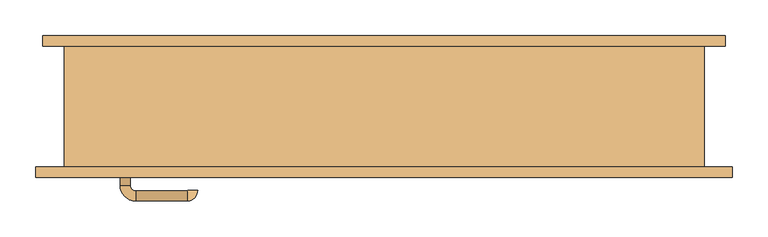
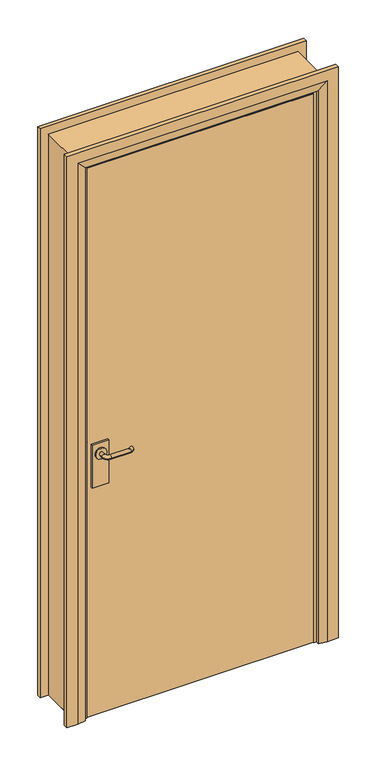
"""IFC4 building model written with IfcOpenShell, lengths in millimetres: door geometry, Porta Simples de Abrir : 80x210cm - Marco de Madeira."""

from ifc_helpers import new_model, si_unit, point, frame, frame_2d, origin, place, context, project, spatial, polyline, circle_curve, ellipse_curve, trimmed, segment, composite_curve, outline, extrude, faceted_brep, source, transform, mapped, element, save
from ifc_brep_helpers import plane_surface, cylinder_surface, revolved_surface, advanced_brep


def door_78011655(model_context):
    return source(origin(), model_context, "Body", "SolidModel", [
        extrude(outline(composite_curve([segment(trimmed(circle_curve(frame_2d((1050.0, -364.0)), 20.0), [point((1050.0, -384.0))], [point((1050.0, -344.0))], False, "CARTESIAN"), True, "CONTINUOUS"), segment(trimmed(circle_curve(frame_2d((1050.0, -364.0)), 20.0), [point((1050.0, -344.0))], [point((1050.0, -384.0))], False, "CARTESIAN"), True, "CONTINUOUS")], self_intersect=False)), frame((0.0, -44.0, 0.0), z_axis=(0.0, 1.0, 0.0), x_axis=(0.0, 0.0, 1.0)), (0.0, 0.0, 1.0), 4.5929895),
        advanced_brep(
        [(-357.0, -39.4070105, 1050.0), (-371.0, -39.4070105, 1050.0), (-357.0, -24.0, 1050.0), (-371.0, -24.0, 1050.0), (-349.0, -2.0, 1050.0), (-349.0, -16.0, 1050.0), (-277.0, -16.0, 1050.0), (-277.0, -2.0, 1050.0), (-276.0, -17.0, 1050.0), (-262.0, -17.0, 1050.0)],
        [
            (0, 1, circle_curve(frame((-364.0, -39.4070105, 1050.0), z_axis=(0.0, -1.0, 0.0), x_axis=(-1.0, 0.0, 0.0)), 7.0)),
            (1, 0, circle_curve(frame((-364.0, -39.4070105, 1050.0), z_axis=(0.0, -1.0, 0.0), x_axis=(-1.0, 0.0, 0.0)), 7.0)),
            (0, 2),
            (2, 3, circle_curve(frame((-364.0, -24.0, 1050.0), z_axis=(0.0, -1.0, 0.0), x_axis=(-1.0, 0.0, 0.0)), 7.0)),
            (3, 1),
            (3, 2, circle_curve(frame((-364.0, -24.0, 1050.0), z_axis=(0.0, -1.0, 0.0), x_axis=(-1.0, 0.0, 0.0)), 7.0)),
            (4, 3, circle_curve(frame((-349.0, -24.0, 1050.0), z_axis=(0.0, 0.0, 1.0), x_axis=(-1.0, 0.0, 0.0)), 22.0)),
            (2, 5, circle_curve(frame((-349.0, -24.0, 1050.0), z_axis=(0.0, 0.0, -1.0), x_axis=(-1.0, 0.0, 0.0)), 8.0)),
            (5, 4, circle_curve(frame((-349.0, -9.0, 1050.0), z_axis=(-1.0, 0.0, 0.0), x_axis=(0.0, 1.0, 0.0)), 7.0)),
            (4, 5, circle_curve(frame((-349.0, -9.0, 1050.0), z_axis=(-1.0, 0.0, 0.0), x_axis=(0.0, 1.0, 0.0)), 7.0)),
            (5, 6),
            (6, 7, circle_curve(frame((-277.0, -9.0, 1050.0), z_axis=(-1.0, 0.0, 0.0), x_axis=(0.0, 1.0, 0.0)), 7.0)),
            (7, 4),
            (7, 6, circle_curve(frame((-277.0, -9.0, 1050.0), z_axis=(-1.0, 0.0, 0.0), x_axis=(0.0, 1.0, 0.0)), 7.0)),
            (8, 9, circle_curve(frame((-269.0, -17.0, 1050.0), z_axis=(0.0, -1.0, 0.0), x_axis=(1.0, 0.0, 0.0)), 7.0)),
            (9, 8, circle_curve(frame((-269.0, -17.0, 1050.0), z_axis=(0.0, -1.0, 0.0), x_axis=(1.0, 0.0, 0.0)), 7.0)),
            (9, 7, circle_curve(frame((-277.0, -17.0, 1050.0), z_axis=(0.0, 0.0, 1.0), x_axis=(0.0, 1.0, 0.0)), 15.0)),
            (6, 8, circle_curve(frame((-277.0, -17.0, 1050.0), z_axis=(0.0, 0.0, -1.0), x_axis=(0.0, 1.0, 0.0)), 1.0)),
        ],
        [
            plane_surface(frame((-364.0, -39.4070105, 1050.0), z_axis=(0.0, -1.0, 0.0), x_axis=(0.0, 0.0, 1.0))),
            cylinder_surface(frame((-364.0, -39.4070105, 1050.0), z_axis=(0.0, -1.0, 0.0), x_axis=(-1.0, 0.0, 0.0)), 7.0),
            revolved_surface(trimmed(ellipse_curve(frame((-364.0, -24.0, 1050.0), z_axis=(0.0, -1.0, 0.0), x_axis=(-1.0, 0.0, 0.0)), 7.0, 7.0), [point((-357.0, -24.0, 1050.0))], [point((-371.0, -24.0, 1050.0))], True, "CARTESIAN"), (-349.0, -24.0, 1050.0), (0.0, 0.0, -1.0)),
            revolved_surface(trimmed(ellipse_curve(frame((-364.0, -24.0, 1050.0), z_axis=(0.0, -1.0, 0.0), x_axis=(-1.0, 0.0, 0.0)), 7.0, 7.0), [point((-371.0, -24.0, 1050.0))], [point((-357.0, -24.0, 1050.0))], True, "CARTESIAN"), (-349.0, -24.0, 1050.0), (0.0, 0.0, -1.0)),
            cylinder_surface(frame((-349.0, -9.0, 1050.0), z_axis=(-1.0, 0.0, 0.0), x_axis=(0.0, 1.0, 0.0)), 7.0),
            plane_surface(frame((-269.0, -17.0, 1050.0), z_axis=(0.0, -1.0, 0.0), x_axis=(0.0, 0.0, 1.0))),
            revolved_surface(trimmed(ellipse_curve(frame((-277.0, -9.0, 1050.0), z_axis=(-1.0, 0.0, 0.0), x_axis=(0.0, 1.0, 0.0)), 7.0, 7.0), [point((-277.0, -16.0, 1050.0))], [point((-277.0, -2.0, 1050.0))], True, "CARTESIAN"), (-277.0, -17.0, 1050.0), (0.0, 0.0, -1.0)),
            revolved_surface(trimmed(ellipse_curve(frame((-277.0, -9.0, 1050.0), z_axis=(-1.0, 0.0, 0.0), x_axis=(0.0, 1.0, 0.0)), 7.0, 7.0), [point((-277.0, -2.0, 1050.0))], [point((-277.0, -16.0, 1050.0))], True, "CARTESIAN"), (-277.0, -17.0, 1050.0), (0.0, 0.0, -1.0)),
        ],
        [
            (0, [[1, 2]]),
            (1, [[-1, 3, 4, 5]]),
            (1, [[-2, -5, 6, -3]]),
            (2, [[7, -4, 8, 9]]),
            (3, [[-8, -6, -7, 10]]),
            (4, [[-9, 11, 12, 13]]),
            (4, [[-10, -13, 14, -11]]),
            (5, [[15, 16]]),
            (6, [[17, -12, 18, -16]]),
            (7, [[-18, -14, -17, -15]]),
        ],
    ),
        extrude(outline(polyline([(-334.0, -50.0), (-394.0, -50.0), (-394.0, -44.0), (-334.0, -44.0), (-334.0, -50.0)])), frame((0.0, 0.0, 925.0), z_axis=(0.0, 0.0, 1.0), x_axis=(1.0, 0.0, 0.0)), (0.0, 0.0, 1.0), 165.0),
        extrude(outline(composite_curve([segment(trimmed(circle_curve(frame_2d((1050.0, -364.0)), 20.0), [point((1050.0, -384.0))], [point((1050.0, -344.0))], False, "CARTESIAN"), True, "CONTINUOUS"), segment(trimmed(circle_curve(frame_2d((1050.0, -364.0)), 20.0), [point((1050.0, -344.0))], [point((1050.0, -384.0))], False, "CARTESIAN"), True, "CONTINUOUS")], self_intersect=False)), frame((0.0, -95.5929895, 0.0), z_axis=(0.0, 1.0, 0.0), x_axis=(0.0, 0.0, 1.0)), (0.0, 0.0, 1.0), 4.5929895),
        advanced_brep(
        [(-357.0, -95.5929895, 1050.0), (-371.0, -95.5929895, 1050.0), (-371.0, -111.0, 1050.0), (-357.0, -111.0, 1050.0), (-349.0, -133.0, 1050.0), (-349.0, -119.0, 1050.0), (-277.0, -133.0, 1050.0), (-277.0, -119.0, 1050.0), (-276.0, -118.0, 1050.0), (-262.0, -118.0, 1050.0)],
        [
            (0, 1, circle_curve(frame((-364.0, -95.5929895, 1050.0), z_axis=(0.0, 1.0, 0.0), x_axis=(-1.0, 0.0, 0.0)), 7.0)),
            (1, 0, circle_curve(frame((-364.0, -95.5929895, 1050.0), z_axis=(0.0, 1.0, 0.0), x_axis=(-1.0, 0.0, 0.0)), 7.0)),
            (1, 2),
            (2, 3, circle_curve(frame((-364.0, -111.0, 1050.0), z_axis=(0.0, 1.0, 0.0), x_axis=(-1.0, 0.0, 0.0)), 7.0)),
            (3, 0),
            (3, 2, circle_curve(frame((-364.0, -111.0, 1050.0), z_axis=(0.0, 1.0, 0.0), x_axis=(-1.0, 0.0, 0.0)), 7.0)),
            (4, 5, circle_curve(frame((-349.0, -126.0, 1050.0), z_axis=(-1.0, 0.0, 0.0), x_axis=(0.0, -1.0, 0.0)), 7.0)),
            (5, 3, circle_curve(frame((-349.0, -111.0, 1050.0), z_axis=(0.0, 0.0, -1.0), x_axis=(-1.0, 0.0, 0.0)), 8.0)),
            (2, 4, circle_curve(frame((-349.0, -111.0, 1050.0), z_axis=(0.0, 0.0, 1.0), x_axis=(-1.0, 0.0, 0.0)), 22.0)),
            (5, 4, circle_curve(frame((-349.0, -126.0, 1050.0), z_axis=(-1.0, 0.0, 0.0), x_axis=(0.0, -1.0, 0.0)), 7.0)),
            (4, 6),
            (6, 7, circle_curve(frame((-277.0, -126.0, 1050.0), z_axis=(-1.0, 0.0, 0.0), x_axis=(0.0, -1.0, 0.0)), 7.0)),
            (7, 5),
            (7, 6, circle_curve(frame((-277.0, -126.0, 1050.0), z_axis=(-1.0, 0.0, 0.0), x_axis=(0.0, -1.0, 0.0)), 7.0)),
            (8, 9, circle_curve(frame((-269.0, -118.0, 1050.0), z_axis=(0.0, 1.0, 0.0), x_axis=(1.0, 0.0, 0.0)), 7.0)),
            (9, 8, circle_curve(frame((-269.0, -118.0, 1050.0), z_axis=(0.0, 1.0, 0.0), x_axis=(1.0, 0.0, 0.0)), 7.0)),
            (8, 7, circle_curve(frame((-277.0, -118.0, 1050.0), z_axis=(0.0, 0.0, -1.0), x_axis=(0.0, -1.0, 0.0)), 1.0)),
            (6, 9, circle_curve(frame((-277.0, -118.0, 1050.0), z_axis=(0.0, 0.0, 1.0), x_axis=(0.0, -1.0, 0.0)), 15.0)),
        ],
        [
            plane_surface(frame((-364.0, -95.5929895, 1050.0), z_axis=(0.0, 1.0, 0.0), x_axis=(0.0, 0.0, 1.0))),
            cylinder_surface(frame((-364.0, -95.5929895, 1050.0), z_axis=(0.0, 1.0, 0.0), x_axis=(-1.0, 0.0, 0.0)), 7.0),
            revolved_surface(trimmed(ellipse_curve(frame((-364.0, -111.0, 1050.0), z_axis=(0.0, -1.0, 0.0), x_axis=(-1.0, 0.0, 0.0)), 7.0, 7.0), [point((-357.0, -111.0, 1050.0))], [point((-371.0, -111.0, 1050.0))], True, "CARTESIAN"), (-349.0, -111.0, 1050.0), (0.0, 0.0, -1.0)),
            revolved_surface(trimmed(ellipse_curve(frame((-364.0, -111.0, 1050.0), z_axis=(0.0, -1.0, 0.0), x_axis=(-1.0, 0.0, 0.0)), 7.0, 7.0), [point((-371.0, -111.0, 1050.0))], [point((-357.0, -111.0, 1050.0))], True, "CARTESIAN"), (-349.0, -111.0, 1050.0), (0.0, 0.0, -1.0)),
            cylinder_surface(frame((-349.0, -126.0, 1050.0), z_axis=(-1.0, 0.0, 0.0), x_axis=(0.0, -1.0, 0.0)), 7.0),
            plane_surface(frame((-269.0, -118.0, 1050.0), z_axis=(0.0, 1.0, 0.0), x_axis=(0.0, 0.0, 1.0))),
            revolved_surface(trimmed(ellipse_curve(frame((-277.0, -126.0, 1050.0), z_axis=(1.0, 0.0, 0.0), x_axis=(0.0, -1.0, 0.0)), 7.0, 7.0), [point((-277.0, -119.0, 1050.0))], [point((-277.0, -133.0, 1050.0))], True, "CARTESIAN"), (-277.0, -118.0, 1050.0), (0.0, 0.0, -1.0)),
            revolved_surface(trimmed(ellipse_curve(frame((-277.0, -126.0, 1050.0), z_axis=(1.0, 0.0, 0.0), x_axis=(0.0, -1.0, 0.0)), 7.0, 7.0), [point((-277.0, -133.0, 1050.0))], [point((-277.0, -119.0, 1050.0))], True, "CARTESIAN"), (-277.0, -118.0, 1050.0), (0.0, 0.0, -1.0)),
        ],
        [
            (0, [[1, 2]]),
            (1, [[3, 4, 5, -2]]),
            (1, [[-5, 6, -3, -1]]),
            (2, [[7, 8, -4, 9]]),
            (3, [[10, -9, -6, -8]]),
            (4, [[11, 12, 13, -7]]),
            (4, [[-13, 14, -11, -10]]),
            (5, [[15, 16]]),
            (6, [[-15, 17, -12, 18]]),
            (7, [[-16, -18, -14, -17]]),
        ],
    ),
        extrude(outline(polyline([(-334.0, -85.0), (-334.0, -91.0), (-394.0, -91.0), (-394.0, -85.0), (-334.0, -85.0)])), frame((0.0, 0.0, 925.0), z_axis=(0.0, 0.0, 1.0), x_axis=(1.0, 0.0, 0.0)), (0.0, 0.0, 1.0), 165.0),
        extrude(outline(polyline([(408.0, -50.0), (408.0, -85.0), (-408.0, -85.0), (-408.0, -50.0), (408.0, -50.0)])), frame((0.0, 0.0, 53.0), z_axis=(0.0, 0.0, 1.0), x_axis=(1.0, 0.0, 0.0)), (0.0, 0.0, 1.0), 2094.0),
        faceted_brep([(480.0, 85.0, 50.0), (410.0, 85.0, 50.0), (410.0, 95.0, 50.0), (440.0, 100.0, 50.0), (480.0, 100.0, 50.0), (480.0, 100.0, 2220.0), (480.0, 85.0, 2220.0), (440.0, 100.0, 2180.0), (-440.0, 100.0, 2180.0), (-440.0, 100.0, 50.0), (-480.0, 100.0, 50.0), (-480.0, 100.0, 2220.0), (410.0, 95.0, 2150.0), (410.0, 85.0, 2150.0), (-480.0, 85.0, 2220.0), (-480.0, 85.0, 50.0), (-410.0, 85.0, 50.0), (-410.0, 85.0, 2150.0), (-410.0, 95.0, 50.0), (-410.0, 95.0, 2150.0)], [[[0, 1, 2, 3, 4]], [[4, 5, 6, 0]], [[3, 7, 8, 9, 10, 11, 5, 4]], [[2, 12, 7, 3]], [[1, 13, 12, 2]], [[0, 6, 14, 15, 16, 17, 13, 1]], [[17, 16, 18, 19]], [[15, 10, 9, 18, 16]], [[11, 10, 15, 14]], [[19, 18, 9, 8]], [[13, 17, 19, 12]], [[5, 11, 14, 6]], [[12, 19, 8, 7]]]),
        faceted_brep([(490.0, -85.0, 50.0), (490.0, -100.0, 50.0), (450.0, -100.0, 50.0), (420.0, -95.0, 50.0), (420.0, -85.0, 50.0), (420.0, -85.0, 2160.0), (-420.0, -85.0, 2160.0), (-420.0, -85.0, 50.0), (-490.0, -85.0, 50.0), (-490.0, -85.0, 2230.0), (490.0, -85.0, 2230.0), (420.0, -95.0, 2160.0), (450.0, -100.0, 2190.0), (490.0, -100.0, 2230.0), (-490.0, -100.0, 2230.0), (-490.0, -100.0, 50.0), (-450.0, -100.0, 50.0), (-450.0, -100.0, 2190.0), (-420.0, -95.0, 50.0), (-420.0, -95.0, 2160.0)], [[[0, 1, 2, 3, 4]], [[4, 5, 6, 7, 8, 9, 10, 0]], [[3, 11, 5, 4]], [[2, 12, 11, 3]], [[1, 13, 14, 15, 16, 17, 12, 2]], [[0, 10, 13, 1]], [[9, 8, 15, 14]], [[8, 7, 18, 16, 15]], [[19, 18, 7, 6]], [[17, 16, 18, 19]], [[11, 19, 6, 5]], [[10, 9, 14, 13]], [[12, 17, 19, 11]]]),
        faceted_brep([(-410.0, -85.0, 50.0), (-450.0, -85.0, 50.0), (-450.0, 85.0, 50.0), (-400.0, 85.0, 50.0), (-400.0, -48.0, 50.0), (-410.0, -48.0, 50.0), (-410.0, -48.0, 2150.0), (-410.0, -85.0, 2150.0), (-400.0, -48.0, 2140.0), (-400.0, 85.0, 2140.0), (-450.0, 85.0, 2190.0), (-450.0, -85.0, 2190.0), (410.0, -85.0, 50.0), (410.0, -48.0, 50.0), (400.0, -48.0, 50.0), (400.0, 85.0, 50.0), (450.0, 85.0, 50.0), (450.0, -85.0, 50.0), (410.0, -85.0, 2150.0), (450.0, -85.0, 2190.0), (450.0, 85.0, 2190.0), (400.0, 85.0, 2140.0), (400.0, -48.0, 2140.0), (410.0, -48.0, 2150.0)], [[[0, 1, 2, 3, 4, 5]], [[5, 6, 7, 0]], [[4, 8, 6, 5]], [[3, 9, 8, 4]], [[2, 10, 9, 3]], [[1, 11, 10, 2]], [[0, 7, 11, 1]], [[12, 13, 14, 15, 16, 17]], [[18, 12, 17, 19]], [[19, 17, 16, 20]], [[20, 16, 15, 21]], [[21, 15, 14, 22]], [[22, 14, 13, 23]], [[23, 13, 12, 18]], [[6, 23, 18, 7]], [[8, 22, 23, 6]], [[9, 21, 22, 8]], [[10, 20, 21, 9]], [[11, 19, 20, 10]], [[7, 18, 19, 11]]]),
        extrude(outline(polyline([(450.0, -50.0), (-450.0, -50.0), (-450.0, 85.0), (450.0, 85.0), (450.0, -50.0)])), frame((0.0, 0.0, 50.0), z_axis=(0.0, 0.0, 1.0), x_axis=(1.0, 0.0, 0.0)), (0.0, 0.0, 1.0), 3.0),
    ])


if __name__ == "__main__":
    model = new_model("IFC4")
    model_context = context("Model", 3, world=origin())
    ifc_project = project(units=[si_unit("LENGTHUNIT", "METRE", prefix="MILLI")], contexts=[model_context])
    site = spatial("IfcSite", under=ifc_project)
    building = spatial("IfcBuilding", under=site)
    placement = place(None, origin())
    door_shape = door_78011655(model_context)
    element("IfcDoor", 1, ObjectType="Porta Simples de Abrir : 80x210cm - Marco de Madeira", at=placement, inside=building, context=model_context, shape_type="MappedRepresentation", body=[
        mapped(door_shape, transform((0.0, 0.0, 0.0), x_axis=(1.0, 0.0, 0.0), y_axis=(0.0, 1.0, 0.0), z_axis=(0.0, 0.0, 1.0))),
    ])
    save(model, "model.ifc")

# Revit data of these elements
# Type "Porta Simples de Abrir : 80x210cm - Marco de Madeira"
#   Type Mark = "P57"
#   SINAPI = ""
#   Analytic Construction = "<Nenhum>"
#   Construction Type = "300"
#   Maçaneta [instance default] = ""
#   Fechadura [instance default] = ""
#   Vão Luz (somente para informação) = 0.780 m
#   Tolerância Folha Vertical = 0.003 m
#   Módulo Básico M = 0.100 m
#   Largura de Coordenação Modular Largura CM = 0.900 m
#   Rough Width = 0.900 m
#   Deslocamento da Horizontal da Folha = 0.000 m
#   Altura de Coordenação Modular Largura CM = 2.200 m
#   Rough Height = 2.200 m
#   Altura Nominal = 2.090 m
#   Ajuste de Coordenação Topo AC Topo = 0.010 m
#   Ajuste de Coordenação Base AC Base = 0.050 m
#   Ajuste de Coordenação AC = 0.010 m
#   Tolerância Folha Horizontal = 0.002 m
#   Largura Folha (somente para informação) = 0.796 m
#   Espessura Folha = 0.035 m
#   Maçaneta - Distância da Folha = 0.044 m
#   Maçaneta - Altura = 1.000 m
#   Largura Nominal (Largura Mn) = 0.820 m
#   Distância do Nível = 0.003 m
#   Aduela Interna Espessura = 0.040 m
#   Aduela Externa Espessura = 0.050 m
#   Altura Folha (somente para informação) = 2.075 m
#   Height = 2.140 m
#   Width = 0.880 m
#   Número de Módulos Básicos nM Largura = 9
#   Número de Módulos Básicos nM Altura = 22
#   Marco Metálico = no
#   Aduela de Madeira = no
#   Aduela Metálica de Canto = no
#   Guarnição Reta = no
#   Guarnição Chanfrada = yes
#   Batente - Material [instance default] = none
#   Painel - Material [instance default] = none
#   Model = ""
#   Function = (empty or 0)
#   Description = (empty or 0)
#   Wall Closure = (empty or 0)
#   Assembly Code = ""
# Element 1 (IfcDoor, "Porta Simples de Abrir : 80x210cm - Marco de Madeira")
#   Materials on its faces: "Porta - Maçaneta", "GRANITO"
# Materials
#   "Porta - Maçaneta": class "Diversos", colour RGB 0 0 0, transparency 0
#   "GRANITO": class "Genérico", colour RGB 120 120 120, transparency 0, Cost = 0
